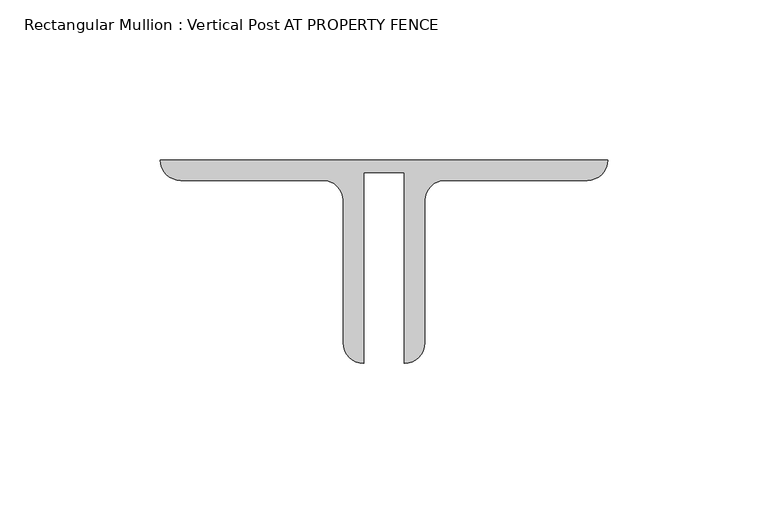
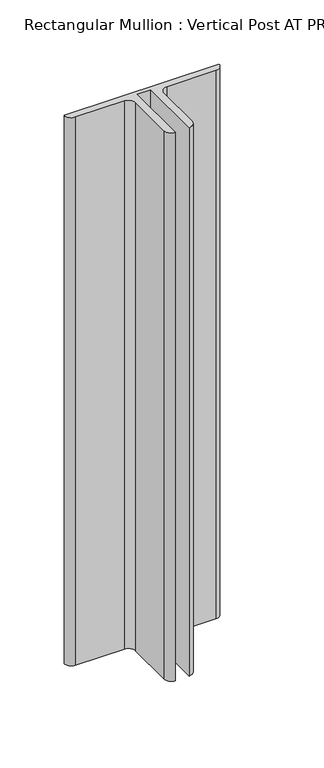
"""IFC4 building model written with IfcOpenShell, lengths in millimetres: member geometry, Rectangular Mullion : Vertical Post AT PROPERTY FENCE."""

from ifc_helpers import new_model, si_unit, point, frame, frame_2d, origin, place, context, project, spatial, polyline, circle_curve, trimmed, segment, composite_curve, outline, extrude, source, transform, mapped, element, save


def rectangular_mullion_vertical_post_at_property_fence_31b97183(model_context):
    return source(origin(), model_context, "Body", "SweptSolid", [
        extrude(outline(composite_curve([segment(polyline([(-63.5, -22.9145205), (-76.2, -22.9145205), (-76.2, -82.55)]), True, "CONTINUOUS"), segment(trimmed(circle_curve(frame_2d((-76.2, -76.2)), 6.35), [point((-76.2, -82.55))], [point((-82.55, -76.2))], False, "CARTESIAN"), True, "CONTINUOUS"), segment(polyline([(-82.55, -76.2), (-82.55, -31.75)]), True, "CONTINUOUS"), segment(trimmed(circle_curve(frame_2d((-88.9, -31.75)), 6.35), [point((-82.55, -31.75))], [point((-88.9, -25.4))], True, "CARTESIAN"), True, "CONTINUOUS"), segment(polyline([(-88.9, -25.4), (-133.35, -25.4)]), True, "CONTINUOUS"), segment(trimmed(circle_curve(frame_2d((-133.35, -19.05)), 6.35), [point((-133.35, -25.4))], [point((-139.7, -19.05))], False, "CARTESIAN"), True, "CONTINUOUS"), segment(polyline([(-139.7, -19.05), (0.0, -19.05)]), True, "CONTINUOUS"), segment(trimmed(circle_curve(frame_2d((-6.35, -19.05)), 6.35), [point((0.0, -19.05))], [point((-6.35, -25.4))], False, "CARTESIAN"), True, "CONTINUOUS"), segment(polyline([(-6.35, -25.4), (-50.8, -25.4)]), True, "CONTINUOUS"), segment(trimmed(circle_curve(frame_2d((-50.8, -31.75)), 6.35), [point((-50.8, -25.4))], [point((-57.15, -31.75))], True, "CARTESIAN"), True, "CONTINUOUS"), segment(polyline([(-57.15, -31.75), (-57.15, -76.2)]), True, "CONTINUOUS"), segment(trimmed(circle_curve(frame_2d((-63.5, -76.2)), 6.35), [point((-57.15, -76.2))], [point((-63.5, -82.55))], False, "CARTESIAN"), True, "CONTINUOUS"), segment(polyline([(-63.5, -82.55), (-63.5, -22.9145205)]), True, "CONTINUOUS")], self_intersect=False)), frame((0.0, 0.0, -522.9663052), z_axis=(0.0, 0.0, 1.0), x_axis=(1.0, 0.0, 0.0)), (0.0, 0.0, 1.0), 522.9663052),
    ])


if __name__ == "__main__":
    model = new_model("IFC4")
    model_context = context("Model", 3, world=origin())
    ifc_project = project(units=[si_unit("LENGTHUNIT", "METRE", prefix="MILLI")], contexts=[model_context])
    site = spatial("IfcSite", under=ifc_project)
    building = spatial("IfcBuilding", under=site)
    placement = place(None, origin())
    rectangular_mullion_vertical_post_at_property_fence_shape = rectangular_mullion_vertical_post_at_property_fence_31b97183(model_context)
    element("IfcMember", 1, ObjectType="Rectangular Mullion : Vertical Post AT PROPERTY FENCE", at=placement, inside=building, context=model_context, shape_type="MappedRepresentation", body=[
        mapped(rectangular_mullion_vertical_post_at_property_fence_shape, transform((0.0, 0.0, 0.0), x_axis=(1.0, 0.0, 0.0), y_axis=(0.0, 1.0, 0.0), z_axis=(0.0, 0.0, 1.0))),
    ])
    save(model, "model.ifc")

# Revit data of these elements
# Type "Rectangular Mullion : Vertical Post AT PROPERTY FENCE"
#   built-in parameter 1007351 = -0.0625 (stored number, unit not read)
#   built-in parameter 1007322 = 0.0126789 (stored number, unit not read)
#   built-in parameter 1007321 = 0.229167 (stored number, unit not read)
#   built-in parameter 1007320 = 0.229167 (stored number, unit not read)
# Element 1 (IfcMember, "Rectangular Mullion : Vertical Post AT PROPERTY FENCE")
#   Materials on its faces: "MAIN FENCE POST: (2) BACK/BACK GALVANIZED ANGLES (2) L2 1/2 X 2 1/2 X 1/4\") ANCHORED TO 8\"W X 42\" DEEP CONCRETE FOOTING(1)"
# Materials
#   "MAIN FENCE POST: (2) BACK/BACK GALVANIZED ANGLES (2) L2 1/2 X 2 1/2 X 1/4\") ANCHORED TO 8\"W X 42\" DEEP CONCRETE FOOTING(1)": class "Unassigned", colour RGB 211 211 211, transparency 0, Cost = 0
